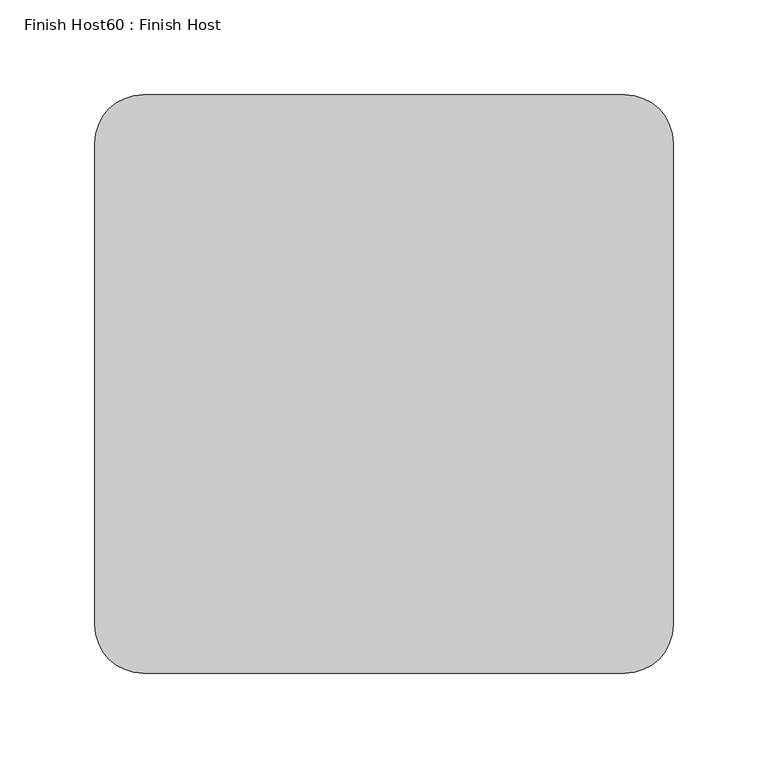
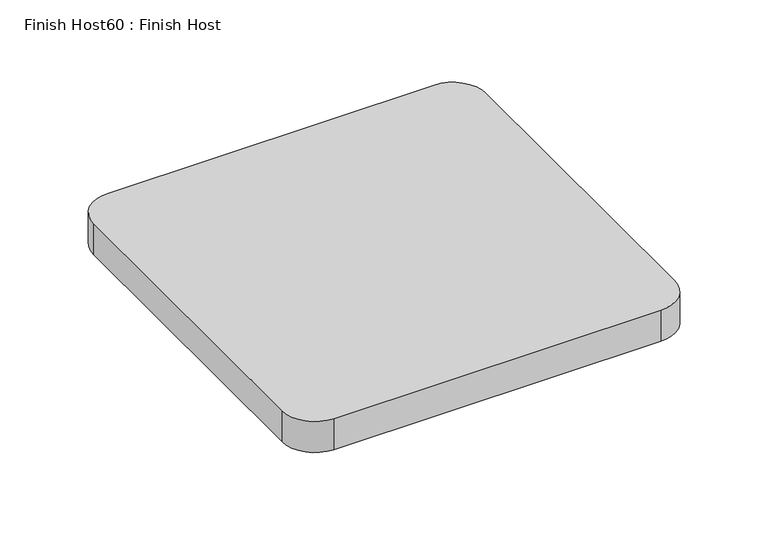
"""IFC4 building model written with IfcOpenShell, lengths in millimetres: proxy geometry, Finish Host60 : Finish Host."""

from ifc_helpers import new_model, si_unit, point, frame_2d, origin, origin_with_axes, place, context, project, spatial, polyline, circle_curve, trimmed, segment, composite_curve, outline, extrude, source, transform, mapped, element, save


def finish_host60_finish_host_390decdd(model_context):
    return source(origin(), model_context, "Body", "SweptSolid", [
        extrude(outline(composite_curve([segment(polyline([(-15309.8939795, 12994.4419385), (-15309.8939795, 13248.4419385)]), True, "CONTINUOUS"), segment(trimmed(circle_curve(frame_2d((-15284.4939795, 13248.4419385)), 25.4), [point((-15309.8939795, 13248.4419385))], [point((-15284.4939795, 13273.8419385))], False, "CARTESIAN"), True, "CONTINUOUS"), segment(polyline([(-15284.4939795, 13273.8419385), (-15030.4939795, 13273.8419385)]), True, "CONTINUOUS"), segment(trimmed(circle_curve(frame_2d((-15030.4939795, 13248.4419385)), 25.4), [point((-15030.4939795, 13273.8419385))], [point((-15005.0939795, 13248.4419385))], False, "CARTESIAN"), True, "CONTINUOUS"), segment(polyline([(-15005.0939795, 13248.4419385), (-15005.0939795, 12994.4419385)]), True, "CONTINUOUS"), segment(trimmed(circle_curve(frame_2d((-15030.4939795, 12994.4419385)), 25.4), [point((-15005.0939795, 12994.4419385))], [point((-15030.4939795, 12969.0419385))], False, "CARTESIAN"), True, "CONTINUOUS"), segment(polyline([(-15030.4939795, 12969.0419385), (-15284.4939795, 12969.0419385)]), True, "CONTINUOUS"), segment(trimmed(circle_curve(frame_2d((-15284.4939795, 12994.4419385)), 25.4), [point((-15284.4939795, 12969.0419385))], [point((-15309.8939795, 12994.4419385))], False, "CARTESIAN"), True, "CONTINUOUS")], self_intersect=False)), origin_with_axes(), (0.0, 0.0, 1.0), 25.4),
    ])


if __name__ == "__main__":
    model = new_model("IFC4")
    model_context = context("Model", 3, world=origin())
    ifc_project = project(units=[si_unit("LENGTHUNIT", "METRE", prefix="MILLI")], contexts=[model_context])
    site = spatial("IfcSite", under=ifc_project)
    building = spatial("IfcBuilding", under=site)
    placement = place(None, origin())
    finish_host60_finish_host_shape = finish_host60_finish_host_390decdd(model_context)
    element("IfcBuildingElementProxy", 1, Name="Finish Host60 : Finish Host", ObjectType="Finish Host60 : Finish Host", at=placement, inside=building, context=model_context, shape_type="MappedRepresentation", body=[
        mapped(finish_host60_finish_host_shape, transform((0.0, 0.0, 0.0), x_axis=(1.0, 0.0, 0.0), y_axis=(0.0, 1.0, 0.0), z_axis=(0.0, 0.0, 1.0))),
    ])
    save(model, "model.ifc")

# Revit data of these elements
# Type "Finish Host60 : Finish Host"
#   Countertop Material = none
# Element 1 (IfcBuildingElementProxy, "Finish Host60 : Finish Host")
#   Materials on its faces: "Thread - Teknion - Forsythia"
# Materials
#   "Thread - Teknion - Forsythia": class "Fabric", colour RGB 204 167 24, transparency 0, Model = "F206", Manufacturer = "Teknion Studio", URL = "http://www.teknion.com/", Description = "Fantasme Full Wool", Cost = 0
